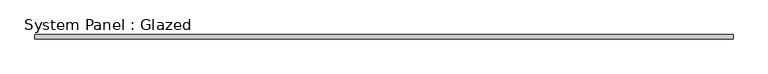
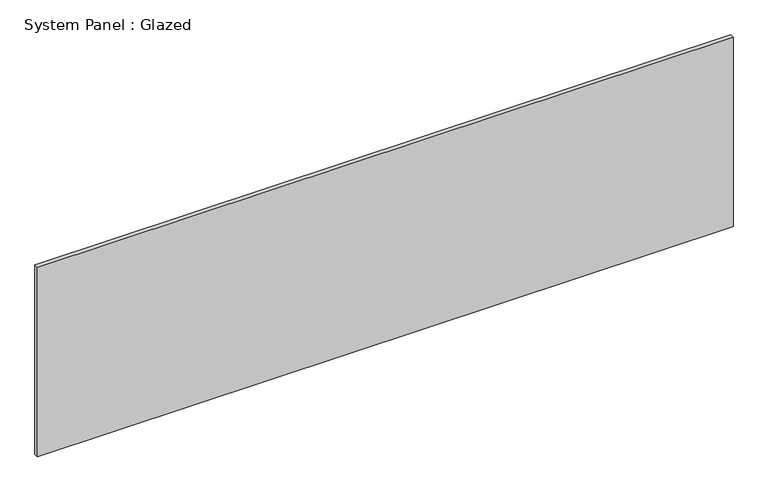
"""IFC4 building model written with IfcOpenShell, lengths in millimetres: plate geometry, System Panel : Glazed."""

from ifc_helpers import new_model, si_unit, origin, origin_with_axes, place, context, project, spatial, polyline, outline, extrude, source, transform, mapped, element, save


def system_panel_glazed_325f688b(model_context):
    return source(origin(), model_context, "Body", "SweptSolid", [
        extrude(outline(polyline([(2082.9545455, 24.5), (-2082.9545455, 24.5), (-2082.9545455, 49.5), (2082.9545455, 49.5), (2082.9545455, 24.5)])), origin_with_axes(), (0.0, 0.0, 1.0), 1200.0),
    ])


if __name__ == "__main__":
    model = new_model("IFC4")
    model_context = context("Model", 3, world=origin())
    ifc_project = project(units=[si_unit("LENGTHUNIT", "METRE", prefix="MILLI")], contexts=[model_context])
    site = spatial("IfcSite", under=ifc_project)
    building = spatial("IfcBuilding", under=site)
    placement = place(None, origin())
    system_panel_glazed_shape = system_panel_glazed_325f688b(model_context)
    element("IfcPlate", 1, ObjectType="System Panel : Glazed", at=placement, inside=building, context=model_context, shape_type="MappedRepresentation", body=[
        mapped(system_panel_glazed_shape, transform((0.0, 0.0, 0.0), x_axis=(1.0, 0.0, 0.0), y_axis=(0.0, 1.0, 0.0), z_axis=(0.0, 0.0, 1.0))),
    ])
    save(model, "model.ifc")

# Revit data of these elements
# Element 1 (IfcPlate, "System Panel : Glazed")
#   Materials on its faces: "Glass"
# Materials
#   "Glass": class "Glass", colour RGB 218 227 224, transparency 0.85, Description = "Soda Lime Glass", Cost = 0
